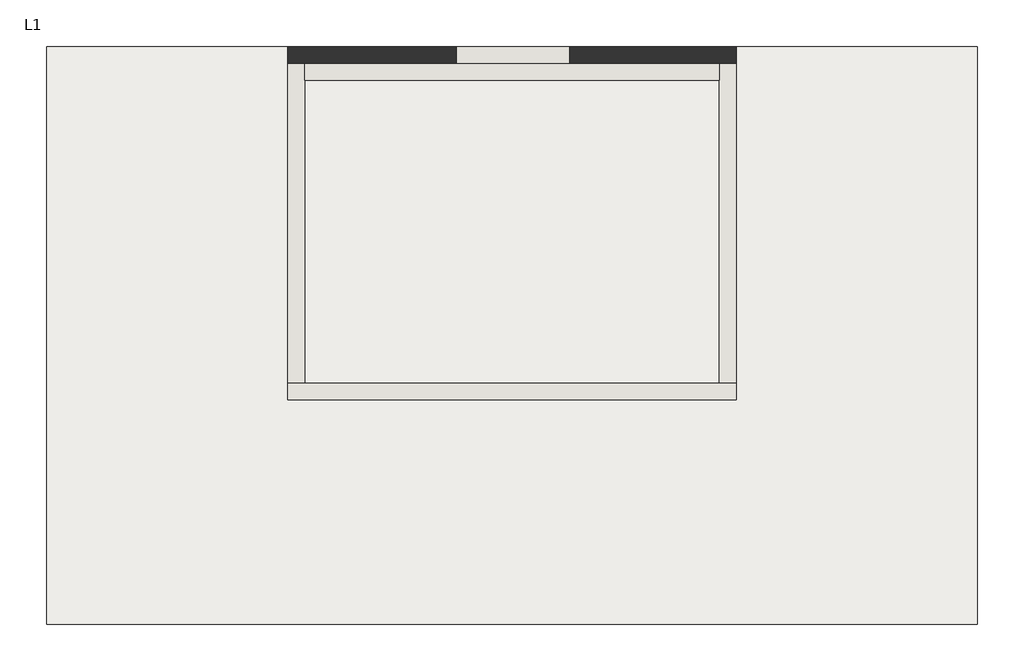
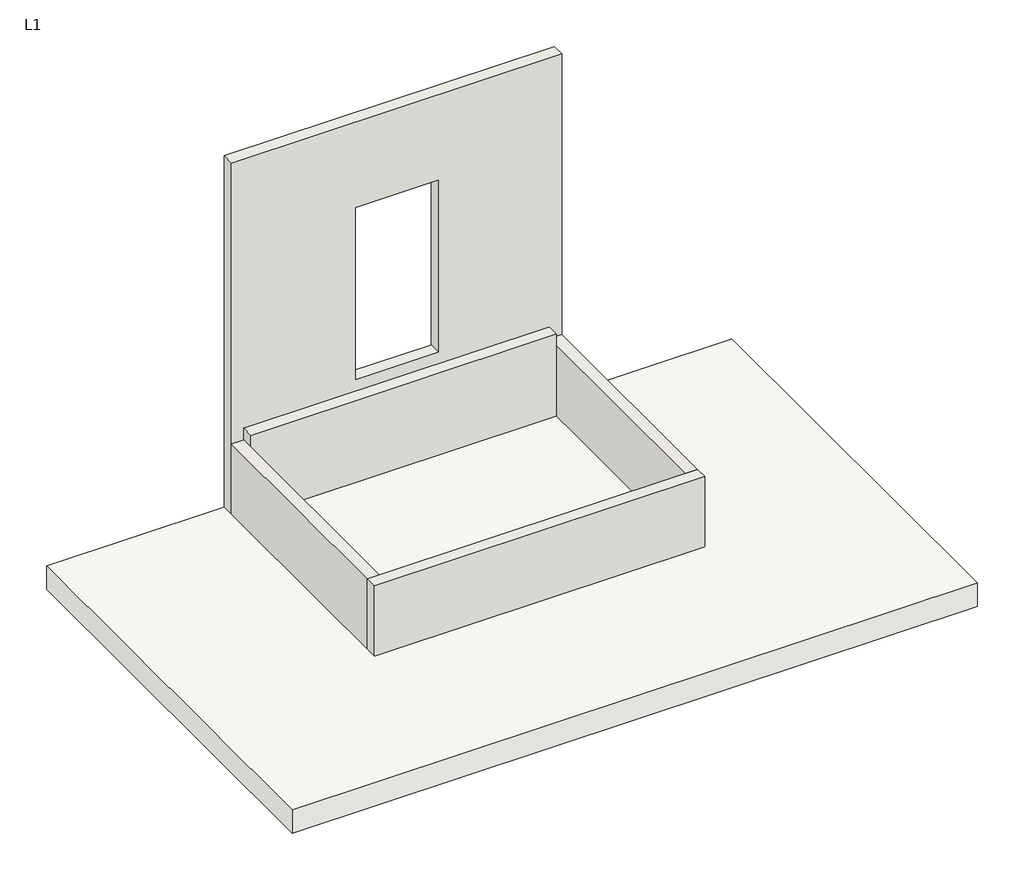
# One storey: 5 walls, 1 slab.
"""IFC4 building model written with IfcOpenShell, lengths in millimetres."""

from ifc_helpers import new_model, si_unit, frame, origin, place, context, project, spatial, polyline, outline, extrude, faceted_brep, element, save

model = new_model("IFC4")

# Units and contexts
model_context = context("Model", 3, world=origin())
ifc_project = project(units=[si_unit("LENGTHUNIT", "METRE", prefix="MILLI")], contexts=[model_context])

# Site, building, storey
site = spatial("IfcSite", under=ifc_project)
building = spatial("IfcBuilding", under=site)
storey = spatial("IfcBuildingStorey", under=building, Name="L1", Elevation=0.0)

# Slab
placement = place(None, origin())
element("IfcSlab", 1, ObjectType="Generic 300mm", at=placement, inside=storey, context=model_context, shape_type="SweptSolid", body=[
    extrude(outline(polyline([(4893.2318, -2858.4292912), (-3406.7682, -2858.4292912), (-3406.7682, 2291.5707088), (4893.2318, 2291.5707088), (4893.2318, -2858.4292912)])), frame((0.0, 0.0, -300.0), z_axis=(0.0, 0.0, 1.0), x_axis=(1.0, 0.0, 0.0)), (0.0, 0.0, 1.0), 300.0),
])

# Walls
element("IfcWall", 2, ObjectType="Generic - 150mm", at=placement, inside=storey, context=model_context, shape_type="Brep", body=[
    faceted_brep([(-1256.7682, -858.4292912, 0.0), (2743.2318, -858.4292912, 0.0), (2743.2318, -858.4292912, 900.0), (-1256.7682, -858.4292912, 900.0), (-1256.7682, -708.4292912, 0.0), (-1256.7682, -708.4292912, 900.0), (-1106.7682, -708.4292912, 900.0), (2593.2318, -708.4292912, 900.0), (2743.2318, -708.4292912, 900.0), (2743.2318, -708.4292912, 0.0), (2593.2318, -708.4292912, 0.0), (-1106.7682, -708.4292912, 0.0)], [[[0, 1, 2, 3]], [[4, 5, 6, 7, 8, 9, 10, 11]], [[1, 0, 4, 11, 10, 9]], [[0, 3, 5, 4]], [[2, 1, 9, 8]], [[3, 2, 8, 7, 6, 5]]]),
])
element("IfcWall", 3, ObjectType="Generic - 150mm", at=placement, inside=storey, context=model_context, shape_type="Brep", body=[
    faceted_brep([(-1106.7682, -708.4292912, 0.0), (-1106.7682, 1991.5707088, 0.0), (-1106.7682, 2141.5707088, 0.0), (-1106.7682, 2141.5707088, 900.0), (-1106.7682, -708.4292912, 900.0), (-1256.7682, -708.4292912, 0.0), (-1256.7682, -708.4292912, 900.0), (-1256.7682, 2141.5707088, 900.0), (-1256.7682, 2141.5707088, 0.0)], [[[0, 1, 2, 3, 4]], [[5, 6, 7, 8]], [[2, 1, 0, 5, 8]], [[4, 3, 7, 6]], [[0, 4, 6, 5]], [[3, 2, 8, 7]]]),
])
element("IfcWall", 4, ObjectType="Generic - 150mm", at=placement, inside=storey, context=model_context, shape_type="Brep", body=[
    faceted_brep([(2743.2318, -708.4292912, 0.0), (2743.2318, 2141.5707088, 0.0), (2743.2318, 2141.5707088, 900.0), (2743.2318, -708.4292912, 900.0), (2593.2318, -708.4292912, 0.0), (2593.2318, -708.4292912, 900.0), (2593.2318, 2141.5707088, 900.0), (2593.2318, 2141.5707088, 0.0), (2593.2318, 1991.5707088, 0.0)], [[[0, 1, 2, 3]], [[4, 5, 6, 7, 8]], [[1, 0, 4, 8, 7]], [[3, 2, 6, 5]], [[0, 3, 5, 4]], [[2, 1, 7, 6]]]),
])
element("IfcWall", 5, ObjectType="Generic - 150mm", at=placement, inside=storey, context=model_context, shape_type="Brep", body=[
    faceted_brep([(-1106.7682, 1991.5707088, 0.0), (2593.2318, 1991.5707088, 0.0), (2593.2318, 1991.5707088, 1050.0), (-1106.7682, 1991.5707088, 1050.0), (-1106.7682, 2141.5707088, 0.0), (-1106.7682, 2141.5707088, 900.0), (-1106.7682, 2141.5707088, 1050.0), (2593.2318, 2141.5707088, 1050.0), (2593.2318, 2141.5707088, 900.0), (2593.2318, 2141.5707088, 0.0)], [[[0, 1, 2, 3]], [[4, 5, 6, 7, 8, 9]], [[1, 0, 4, 9]], [[3, 2, 7, 6]], [[0, 3, 6, 5, 4]], [[2, 1, 9, 8, 7]]]),
])
element("IfcWall", 6, ObjectType="Generic - 150mm", at=placement, inside=storey, context=model_context, shape_type="SweptSolid", body=[
    extrude(outline(polyline([(0.0, -1256.7682), (0.0, 2743.2318), (4500.0, 2743.2318), (4500.0, -1256.7682), (0.0, -1256.7682)]), holes=[polyline([(1200.0, 252.7568), (3400.0, 252.7568), (3400.0, 1252.7568), (1200.0, 1252.7568), (1200.0, 252.7568)])]), frame((0.0, 2141.5707088, 0.0), z_axis=(0.0, 1.0, 0.0), x_axis=(0.0, 0.0, 1.0)), (0.0, 0.0, 1.0), 150.0),
])

save(model, "model.ifc")

# Revit data of these elements
# Project information
#   Название организации = "Organization Name"
#   Описание организации = "Organization Description"
#   Наименование здания = "Building Name"
#   Дата утверждения проекта = "Issue Date"
#   Статус проекта = "Project Status"
#   Заказчик = "Client Name"
#   Адрес проекта = "Enter address here\nAddress Line 2"
#   Наименование проекта = "Project Name"
#   Номер проекта = "Project Number"
# Type "Generic 300mm"
#   Description = "Generic Floor (Material By Category), 300mm thick"
#   Function = 0
#   Layers, outside or top first: 300 mm no material (function 1)
# Type "Generic - 150mm"
#   Description = "Generic Wall (Material By Category), 150mm thick"
#   Type Mark = "G04"
#   Layers, outside or top first: 150 mm no material (function 1)
# Element 1 (IfcSlab, "Generic 300mm")
#   Height Offset From Level = 0 mm
#   Phase Created = New Construction
#   Materials on its faces: "Default Floor"
# Element 2 (IfcWall, "Generic - 150mm")
#   Top Offset = 0 mm
#   Base Offset = 0 mm
#   wall height = 1200 mm
#   Phase Created = New Construction
#   Base Constraint = L1
#   Top Constraint = L2
#   Materials on its faces: "Default Wall"
# Elements 3, 4 (IfcWall, "Generic - 150mm")
#   Top Offset = 0 mm
#   Base Offset = 0 mm
#   Unconnected Height = 900 mm
#   wall height = 900 mm
#   Phase Created = New Construction
#   Base Constraint = L1
#   Materials on its faces: "Default Wall"
# Element 5 (IfcWall, "Generic - 150mm")
#   Top Offset = 0 mm
#   Base Offset = 0 mm
#   Unconnected Height = 1050 mm
#   wall height = 1050 mm
#   Phase Created = New Construction
#   Base Constraint = L1
#   Materials on its faces: "Default Wall"
# Element 6 (IfcWall, "Generic - 150mm")
#   Top Offset = 0 mm
#   Base Offset = 0 mm
#   Unconnected Height = 4500 mm
#   wall height = 4500 mm
#   Phase Created = New Construction
#   Base Constraint = L1
#   Materials on its faces: "Default Wall"
# Materials
#   "Default Floor": class "Miscellaneous", colour RGB 128 128 128, transparency 0, Cost = 0
#   "Default Wall": class "Miscellaneous", colour RGB 192 192 192, transparency 0, Cost = 0
